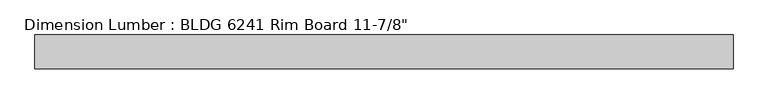
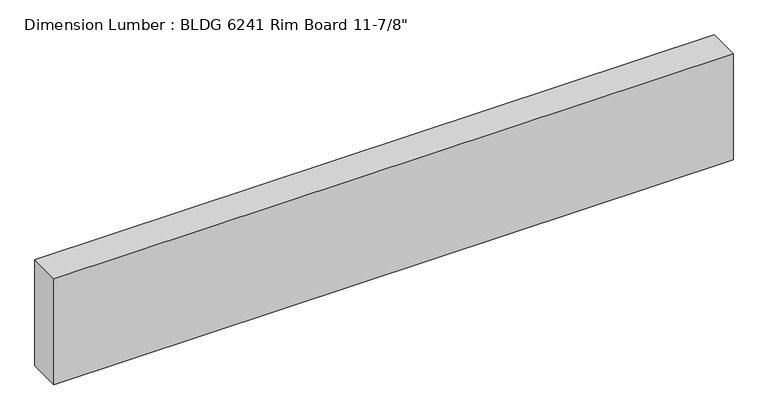
"""IFC4 building model written with IfcOpenShell, lengths in millimetres: beam geometry."""

from ifc_helpers import new_model, si_unit, frame, origin, place, context, project, spatial, polyline, outline, extrude, source, transform, mapped, element, save


def beam_b5369756(model_context):
    return source(origin(), model_context, "Body", "SweptSolid", [
        extrude(outline(polyline([(914.4, 44.45), (914.4, -44.45), (-914.4, -44.45), (-914.4, 44.45), (914.4, 44.45)])), frame((0.0, 0.0, -150.8125), z_axis=(0.0, 0.0, 1.0), x_axis=(1.0, 0.0, 0.0)), (0.0, 0.0, 1.0), 301.625),
    ])


if __name__ == "__main__":
    model = new_model("IFC4")
    model_context = context("Model", 3, world=origin())
    ifc_project = project(units=[si_unit("LENGTHUNIT", "METRE", prefix="MILLI")], contexts=[model_context])
    site = spatial("IfcSite", under=ifc_project)
    building = spatial("IfcBuilding", under=site)
    placement = place(None, origin())
    beam_shape = beam_b5369756(model_context)
    element("IfcBeam", 1, ObjectType="Dimension Lumber : BLDG 6241 Rim Board 11-7/8\"", at=placement, inside=building, context=model_context, shape_type="MappedRepresentation", body=[
        mapped(beam_shape, transform((0.0, 0.0, 0.0), x_axis=(1.0, 0.0, 0.0), y_axis=(0.0, 1.0, 0.0), z_axis=(0.0, 0.0, 1.0))),
    ])
    save(model, "model.ifc")

# Revit data of these elements
# Type "Dimension Lumber : BLDG 6241 Rim Board 11-7/8\""
#   Assembly Code = "B10"
#   A = 0.273472 SF
#   Length [instance default] = 5' - 0"
#   b = 0' - 3 1/2"
#   d = 0' - 11 7/8"
#   Structural Material [instance default] = Softwood, Lumber
# Element 1 (IfcBeam, "Dimension Lumber : BLDG 6241 Rim Board 11-7/8\"")
#   Materials on its faces: "Softwood, Lumber"
# Materials
#   "Softwood, Lumber": class "Wood", colour RGB 223 192 134, transparency 0, Description = "Pinus Echinata", Cost = 0
